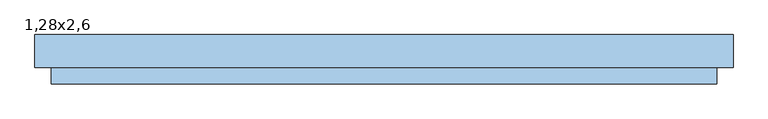
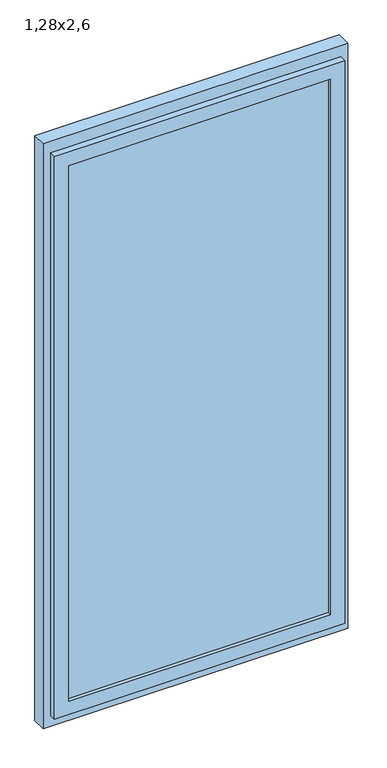
"""IFC4 building model written with IfcOpenShell, lengths in millimetres: window geometry, Fenstertür 1-flg : 1,28x2,6."""

from ifc_helpers import new_model, si_unit, frame, origin, place, context, project, spatial, polyline, outline, extrude, faceted_brep, source, transform, mapped, element, save


def window_1_28x2_6_953aa5e8(model_context):
    return source(origin(), model_context, "Body", "SolidModel", [
        extrude(outline(polyline([(2600.0, 640.0), (2600.0, -640.0), (0.0, -640.0), (0.0, 640.0), (2600.0, 640.0)]), holes=[polyline([(2520.0, 580.0), (80.0, 580.0), (80.0, -580.0), (2520.0, -580.0), (2520.0, 580.0)])]), frame((0.0, 20.0, 0.0), z_axis=(0.0, 1.0, 0.0), x_axis=(0.0, 0.0, 1.0)), (0.0, 0.0, 1.0), 60.0),
        faceted_brep([(610.0, 20.0, 2550.0), (610.0, -10.0, 2550.0), (610.0, -10.0, 50.0), (610.0, 20.0, 50.0), (-610.0, -10.0, 2550.0), (-610.0, -10.0, 50.0), (550.0, -10.0, 110.0), (-550.0, -10.0, 110.0), (-550.0, -10.0, 2490.0), (550.0, -10.0, 2490.0), (-610.0, 20.0, 50.0), (-610.0, 20.0, 2550.0), (580.0, 20.0, 2520.0), (-580.0, 20.0, 2520.0), (-580.0, 20.0, 80.0), (580.0, 20.0, 80.0), (580.0, 50.0, 2520.0), (580.0, 50.0, 80.0), (-580.0, 50.0, 80.0), (-580.0, 50.0, 2520.0), (550.0, 50.0, 2490.0), (-550.0, 50.0, 2490.0), (-550.0, 50.0, 110.0), (550.0, 50.0, 110.0)], [[[0, 1, 2, 3]], [[1, 4, 5, 2], [6, 7, 8, 9]], [[3, 2, 5, 10]], [[3, 10, 11, 0], [12, 13, 14, 15]], [[16, 12, 15, 17]], [[17, 15, 14, 18]], [[17, 18, 19, 16], [20, 21, 22, 23]], [[9, 20, 23, 6]], [[6, 23, 22, 7]], [[10, 5, 4, 11]], [[18, 14, 13, 19]], [[7, 22, 21, 8]], [[11, 4, 1, 0]], [[19, 13, 12, 16]], [[8, 21, 20, 9]]]),
        extrude(outline(polyline([(550.0, 5.0), (-550.0, 5.0), (-550.0, 35.0), (550.0, 35.0), (550.0, 5.0)])), frame((0.0, 0.0, 110.0), z_axis=(0.0, 0.0, 1.0), x_axis=(1.0, 0.0, 0.0)), (0.0, 0.0, 1.0), 2380.0),
    ])


if __name__ == "__main__":
    model = new_model("IFC4")
    model_context = context("Model", 3, world=origin())
    ifc_project = project(units=[si_unit("LENGTHUNIT", "METRE", prefix="MILLI")], contexts=[model_context])
    site = spatial("IfcSite", under=ifc_project)
    building = spatial("IfcBuilding", under=site)
    placement = place(None, origin())
    window_1_28x2_6_shape = window_1_28x2_6_953aa5e8(model_context)
    element("IfcWindow", 1, ObjectType="Fenstertür 1-flg : 1,28x2,6", at=placement, inside=building, context=model_context, shape_type="MappedRepresentation", body=[
        mapped(window_1_28x2_6_shape, transform((0.0, 0.0, 0.0), x_axis=(1.0, 0.0, 0.0), y_axis=(0.0, 1.0, 0.0), z_axis=(0.0, 0.0, 1.0))),
    ])
    save(model, "model.ifc")

# Revit data of these elements
# Type "Fenstertür 1-flg : 1,28x2,6"
#   Type Mark = "65"
#   Operation = "SinglePanel"
#   Construction Type Id = "GSP4R"
#   Keynote = "16.05.01"
#   Analytic Construction = "1/8 Zoll Pilkington-Verglasung einfach"
#   Visual Light Transmittance = 0.9
#   Thermal Resistance (R) = 0.1491 (m²·K)/W
#   Solar Heat Gain Coefficient = 0.86
#   Rough Width = 1.280 m
#   Rough Height = 2.600 m
#   Heat Transfer Coefficient (U) = 6.7069 W/(m²·K)
#   Rahmentiefe = 0.060 m
#   Rahmenhöhe - unten = 0.080 m
#   Rahmenhöhe - oben = 0.080 m
#   Rahmenbreite = 0.060 m
#   Height = 2.600 m
#   Tiefe Flügel = 0.060 m
#   Flügelbreite = 0.060 m
#   Einbautiefe (von außen) [instance default] = 0.080 m
#   Width = 1.280 m
#   Kippflügel [instance default] = yes
#   Drehflügel im Grundriss darstellen [instance default] = yes
#   Drehflügel 1 [instance default] = yes
#   Rahmen 1 [instance default] = none
#   Glas [instance default] = none
#   Flügel [instance default] = none
#   Fensterbank Außenseite [instance default] = none
#   Wall Closure = (empty or 0)
# Element 1 (IfcWindow, "Fenstertür 1-flg : 1,28x2,6")
#   Einbautiefe (von außen) = 0.230 m
#   Materials on its faces: "Kunststoff - Weiß", "Glas"
# Materials
#   "Kunststoff - Weiß": class "Kunststoff", colour RGB 249 249 249, transparency 0, Cost = 0
#   "Glas": class "Glas", colour RGB 0 0 255, transparency 0.75, Comments = "Render-Darstellung nicht aktualisiert ", Cost = 0
